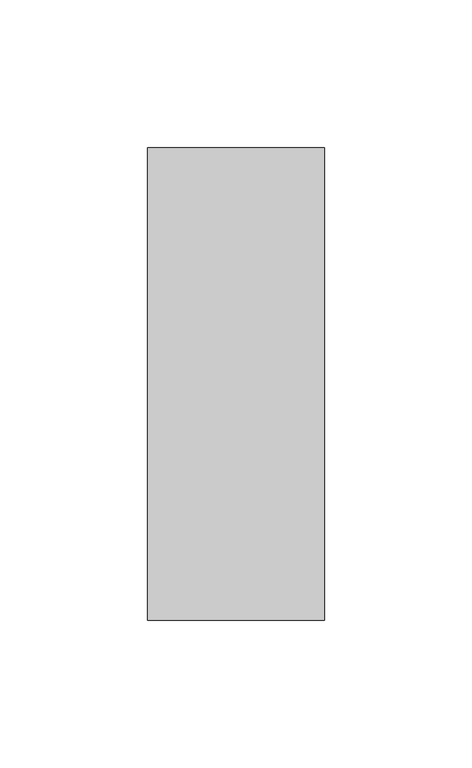
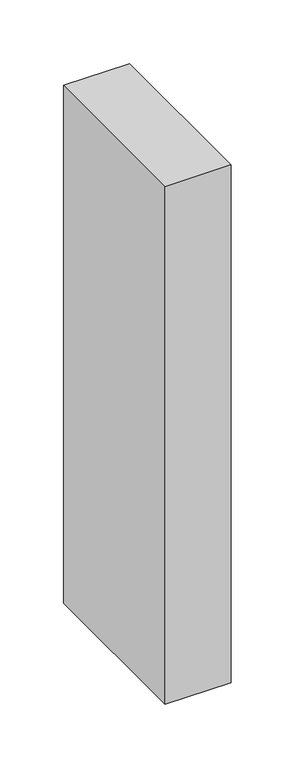
"""IFC4 building model written with IfcOpenShell, lengths in millimetres: column geometry, Madeira de lei-Coluna : Pontalete 6X16cm."""

from ifc_helpers import new_model, si_unit, frame, origin, place, context, project, spatial, polyline, outline, extrude, source, transform, mapped, element, save


def column_924cc83b(model_context):
    return source(origin(), model_context, "Body", "SweptSolid", [
        extrude(outline(polyline([(30.0, 80.0), (30.0, -80.0), (-30.0, -80.0), (-30.0, 80.0), (30.0, 80.0)])), frame((0.0, 0.0, 4460.0), z_axis=(0.0, 0.0, 1.0), x_axis=(1.0, 0.0, 0.0)), (0.0, 0.0, 1.0), 497.0),
    ])


if __name__ == "__main__":
    model = new_model("IFC4")
    model_context = context("Model", 3, world=origin())
    ifc_project = project(units=[si_unit("LENGTHUNIT", "METRE", prefix="MILLI")], contexts=[model_context])
    site = spatial("IfcSite", under=ifc_project)
    building = spatial("IfcBuilding", under=site)
    placement = place(None, origin())
    column_shape = column_924cc83b(model_context)
    element("IfcColumn", 1, ObjectType="Madeira de lei-Coluna : Pontalete 6X16cm", at=placement, inside=building, context=model_context, shape_type="MappedRepresentation", body=[
        mapped(column_shape, transform((0.0, 0.0, 0.0), x_axis=(1.0, 0.0, 0.0), y_axis=(0.0, 1.0, 0.0), z_axis=(0.0, 0.0, 1.0))),
    ])
    save(model, "model.ifc")

# Revit data of these elements
# Type "Madeira de lei-Coluna : Pontalete 6X16cm"
#   A = 0.01952 m²
#   b = 0.06 m
#   d = 0.16 m
#   Structural Material [instance default] = none
#   Assembly Code = ""
# Element 1 (IfcColumn, "Madeira de lei-Coluna : Pontalete 6X16cm")
#   Structural Material = .MADEIRAMENTO
#   Materials on its faces: ".MADEIRAMENTO"
# Materials
#   ".MADEIRAMENTO": class ".CC_MADEIRAS", colour RGB 212 179 113, transparency 0, Cost = 0
